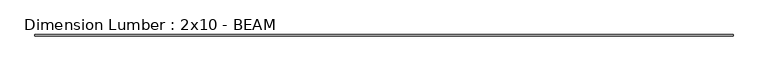
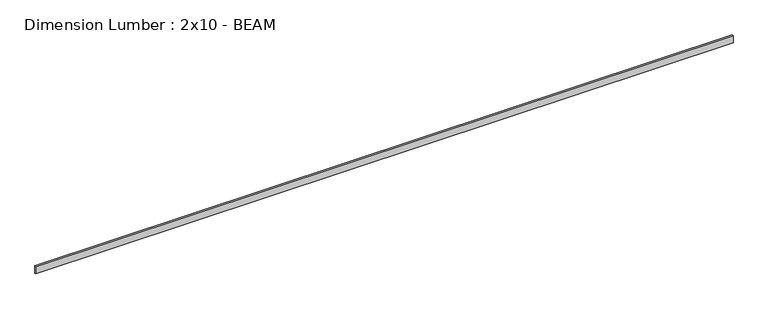
"""IFC4 building model written with IfcOpenShell, lengths in millimetres: beam geometry, Dimension Lumber : 2x10 - BEAM."""

from ifc_helpers import new_model, si_unit, frame, origin, place, context, project, spatial, polyline, outline, extrude, source, transform, mapped, element, save


def dimension_lumber_2x10_beam_4c1f0bd3(model_context):
    return source(origin(), model_context, "Body", "SweptSolid", [
        extrude(outline(polyline([(10487.6663185, 19.05), (10487.6663185, -19.05), (-10791.1836815, -19.05), (-10791.1836815, 19.05), (10487.6663185, 19.05)])), frame((0.0, 0.0, -117.475), z_axis=(0.0, 0.0, 1.0), x_axis=(1.0, 0.0, 0.0)), (0.0, 0.0, 1.0), 234.95),
    ])


if __name__ == "__main__":
    model = new_model("IFC4")
    model_context = context("Model", 3, world=origin())
    ifc_project = project(units=[si_unit("LENGTHUNIT", "METRE", prefix="MILLI")], contexts=[model_context])
    site = spatial("IfcSite", under=ifc_project)
    building = spatial("IfcBuilding", under=site)
    placement = place(None, origin())
    dimension_lumber_2x10_beam_shape = dimension_lumber_2x10_beam_4c1f0bd3(model_context)
    element("IfcBeam", 1, ObjectType="Dimension Lumber : 2x10 - BEAM", at=placement, inside=building, context=model_context, shape_type="MappedRepresentation", body=[
        mapped(dimension_lumber_2x10_beam_shape, transform((0.0, 0.0, 0.0), x_axis=(1.0, 0.0, 0.0), y_axis=(0.0, 1.0, 0.0), z_axis=(0.0, 0.0, 1.0))),
    ])
    save(model, "model.ifc")

# Revit data of these elements
# Type "Dimension Lumber : 2x10 - BEAM"
#   Assembly Code = "B10"
#   A = 0.0755556 SF
#   Length [instance default] = 5' - 0"
#   b = 0' - 1 1/2"
#   d = 0' - 9 1/4"
#   Structural Material = (3) SISTERED 2X10s AT BEAM
# Element 1 (IfcBeam, "Dimension Lumber : 2x10 - BEAM")
#   Materials on its faces: "(3) SISTERED 2X10s AT BEAM"
# Materials
#   "(3) SISTERED 2X10s AT BEAM": class "Wood", colour RGB 234 198 147, transparency 0, Description = "Pinus Echinata", Cost = 0
